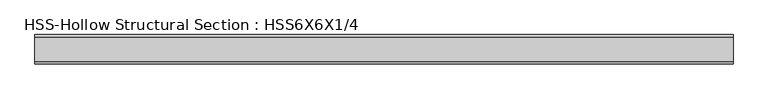
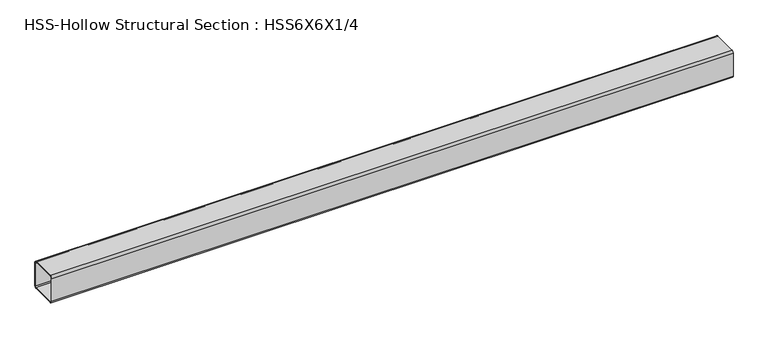
"""IFC4 building model written with IfcOpenShell, lengths in millimetres: beam geometry, HSS-Hollow Structural Section : HSS6X6X1/4."""

from ifc_helpers import new_model, si_unit, point, frame, frame_2d, origin, place, context, project, spatial, polyline, circle_curve, trimmed, segment, composite_curve, outline, extrude, source, transform, mapped, element, save


def hss_hollow_structural_section_hss6x6x1_4_80d8be0f(model_context):
    return source(origin(), model_context, "Body", "SweptSolid", [
        extrude(outline(composite_curve([segment(polyline([(76.2, 64.3636), (76.2, -64.3636)]), True, "CONTINUOUS"), segment(trimmed(circle_curve(frame_2d((64.3636, -64.3636)), 11.8364), [point((76.2, -64.3636))], [point((64.3636, -76.2))], False, "CARTESIAN"), True, "CONTINUOUS"), segment(polyline([(64.3636, -76.2), (-64.3636, -76.2)]), True, "CONTINUOUS"), segment(trimmed(circle_curve(frame_2d((-64.3636, -64.3636)), 11.8364), [point((-64.3636, -76.2))], [point((-76.2, -64.3636))], False, "CARTESIAN"), True, "CONTINUOUS"), segment(polyline([(-76.2, -64.3636), (-76.2, 64.3636)]), True, "CONTINUOUS"), segment(trimmed(circle_curve(frame_2d((-64.3636, 64.3636)), 11.8364), [point((-76.2, 64.3636))], [point((-64.3636, 76.2))], False, "CARTESIAN"), True, "CONTINUOUS"), segment(polyline([(-64.3636, 76.2), (64.3636, 76.2)]), True, "CONTINUOUS"), segment(trimmed(circle_curve(frame_2d((64.3636, 64.3636)), 11.8364), [point((64.3636, 76.2))], [point((76.2, 64.3636))], False, "CARTESIAN"), True, "CONTINUOUS")], self_intersect=False), holes=[composite_curve([segment(trimmed(circle_curve(frame_2d((-64.3636, 64.3636)), 5.9182), [point((-64.3636, 70.2818))], [point((-70.2818, 64.3636))], True, "CARTESIAN"), True, "CONTINUOUS"), segment(polyline([(-70.2818, 64.3636), (-70.2818, -64.3636)]), True, "CONTINUOUS"), segment(trimmed(circle_curve(frame_2d((-64.3636, -64.3636)), 5.9182), [point((-70.2818, -64.3636))], [point((-64.3636, -70.2818))], True, "CARTESIAN"), True, "CONTINUOUS"), segment(polyline([(-64.3636, -70.2818), (64.3636, -70.2818)]), True, "CONTINUOUS"), segment(trimmed(circle_curve(frame_2d((64.3636, -64.3636)), 5.9182), [point((64.3636, -70.2818))], [point((70.2818, -64.3636))], True, "CARTESIAN"), True, "CONTINUOUS"), segment(polyline([(70.2818, -64.3636), (70.2818, 64.3636)]), True, "CONTINUOUS"), segment(trimmed(circle_curve(frame_2d((64.3636, 64.3636)), 5.9182), [point((70.2818, 64.3636))], [point((64.3636, 70.2818))], True, "CARTESIAN"), True, "CONTINUOUS"), segment(polyline([(64.3636, 70.2818), (-64.3636, 70.2818)]), True, "CONTINUOUS")], self_intersect=False)]), frame((-1816.3233784, 0.0, 0.0), z_axis=(1.0, 0.0, 0.0), x_axis=(0.0, 1.0, 0.0)), (0.0, 0.0, 1.0), 3632.6467568),
    ])


if __name__ == "__main__":
    model = new_model("IFC4")
    model_context = context("Model", 3, world=origin())
    ifc_project = project(units=[si_unit("LENGTHUNIT", "METRE", prefix="MILLI")], contexts=[model_context])
    site = spatial("IfcSite", under=ifc_project)
    building = spatial("IfcBuilding", under=site)
    placement = place(None, origin())
    hss_hollow_structural_section_hss6x6x1_4_shape = hss_hollow_structural_section_hss6x6x1_4_80d8be0f(model_context)
    element("IfcBeam", 1, ObjectType="HSS-Hollow Structural Section : HSS6X6X1/4", at=placement, inside=building, context=model_context, shape_type="MappedRepresentation", body=[
        mapped(hss_hollow_structural_section_hss6x6x1_4_shape, transform((0.0, 0.0, 0.0), x_axis=(1.0, 0.0, 0.0), y_axis=(0.0, 1.0, 0.0), z_axis=(0.0, 0.0, 1.0))),
    ])
    save(model, "model.ifc")

# Revit data of these elements
# Type "HSS-Hollow Structural Section : HSS6X6X1/4"
#   Assembly Code = "B10"
#   Shape = "Square"
#   W = 19
#   Ht = 0' - 6"
#   Length [instance default] = 5' - 0"
#   b = 0' - 6"
#   kr = 0' - 0.466"
#   t = 0' - 0.233"
#   A = 0.0363889 SF
#   Structural Material [instance default] = Steel ASTM A500, Grade B, Rectangular and Square
# Element 1 (IfcBeam, "HSS-Hollow Structural Section : HSS6X6X1/4")
#   Materials on its faces: "Steel ASTM A500, Grade B, Rectangular and Square"
# Materials
#   "Steel ASTM A500, Grade B, Rectangular and Square": class "Metal", colour RGB 199 199 199, transparency 0, Description = "Carbon steel", Cost = 0
